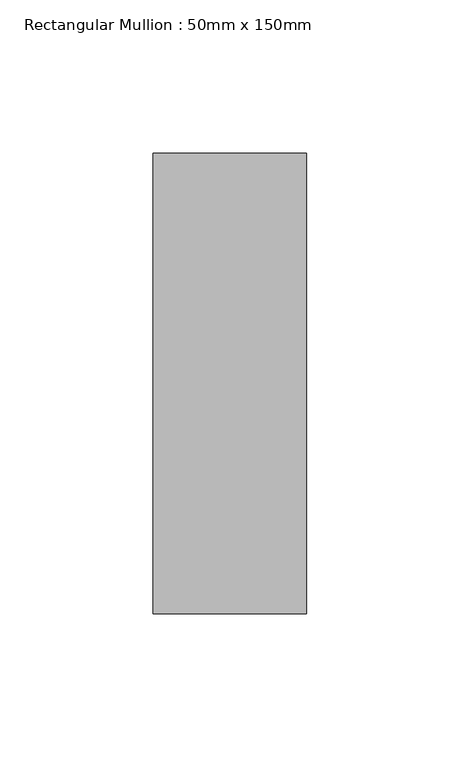
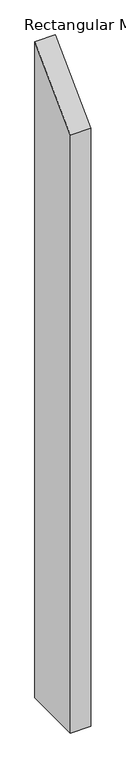
"""IFC4 building model written with IfcOpenShell, lengths in millimetres: member geometry, Rectangular Mullion : 50mm x 150mm."""

from ifc_helpers import new_model, si_unit, frame, origin, place, context, project, spatial, polyline, outline, extrude, source, transform, mapped, element, save


def rectangular_mullion_50mm_x_150mm_ebdf0d5b(model_context):
    return source(origin(), model_context, "Body", "SweptSolid", [
        extrude(outline(polyline([(-75.0, -75.0), (75.0, 75.0), (75.0, -1615.6357052), (-75.0, -1615.6357052), (-75.0, -75.0)])), frame((-50.0, 0.0, 0.0), z_axis=(1.0, 0.0, 0.0), x_axis=(0.0, 1.0, 0.0)), (0.0, 0.0, 1.0), 50.0),
    ])


if __name__ == "__main__":
    model = new_model("IFC4")
    model_context = context("Model", 3, world=origin())
    ifc_project = project(units=[si_unit("LENGTHUNIT", "METRE", prefix="MILLI")], contexts=[model_context])
    site = spatial("IfcSite", under=ifc_project)
    building = spatial("IfcBuilding", under=site)
    placement = place(None, origin())
    rectangular_mullion_50mm_x_150mm_shape = rectangular_mullion_50mm_x_150mm_ebdf0d5b(model_context)
    element("IfcMember", 1, ObjectType="Rectangular Mullion : 50mm x 150mm", at=placement, inside=building, context=model_context, shape_type="MappedRepresentation", body=[
        mapped(rectangular_mullion_50mm_x_150mm_shape, transform((0.0, 0.0, 0.0), x_axis=(1.0, 0.0, 0.0), y_axis=(0.0, 1.0, 0.0), z_axis=(0.0, 0.0, 1.0))),
    ])
    save(model, "model.ifc")

# Revit data of these elements
# Type "Rectangular Mullion : 50mm x 150mm"
#   built-in parameter 1007304 = 0.492126 (stored number, unit not read)
#   built-in parameter 1007301 = 0.082021 (stored number, unit not read)
#   built-in parameter 1007300 = 0.082021 (stored number, unit not read)
# Element 1 (IfcMember, "Rectangular Mullion : 50mm x 150mm")
#   Materials on its faces: "Aluminum"
# Materials
#   "Aluminum": class "Metal", colour RGB 244 244 244, transparency 0, Description = "Aluminum 6061", Cost = 0
